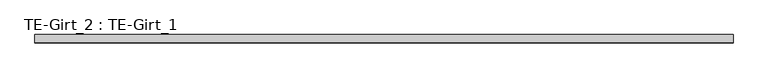
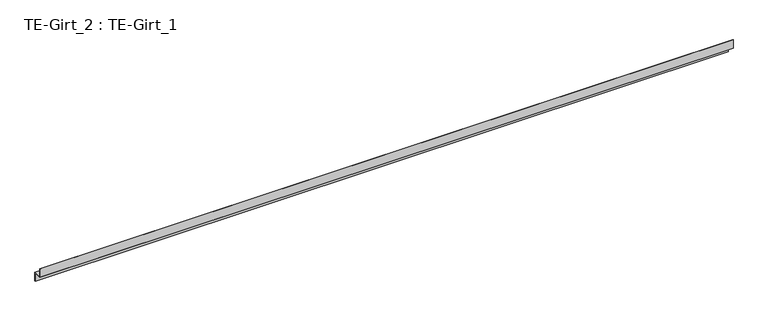
"""IFC4 building model written with IfcOpenShell, lengths in millimetres: proxy geometry, TE-Girt_2 : TE-Girt_1."""

from ifc_helpers import new_model, si_unit, frame, origin, place, context, project, spatial, polyline, outline, extrude, source, transform, mapped, element, save


def te_girt_2_te_girt_1_d8d35839(model_context):
    return source(origin(), model_context, "Body", "SweptSolid", [
        extrude(outline(polyline([(-531639.2163841, 1657.35), (-531639.2163841, 1619.25), (-531640.1093528, 1619.25), (-531640.1093528, 1656.4570312), (-531674.1249348, 1656.4570312), (-531674.1249348, 1694.5570312), (-531673.231966, 1694.5570312), (-531673.231966, 1657.35), (-531639.2163841, 1657.35)])), frame((587397.6434739, 0.0, 0.0), z_axis=(1.0, 0.0, 0.0), x_axis=(0.0, 1.0, 0.0)), (0.0, 0.0, 1.0), 2921.0),
    ])


if __name__ == "__main__":
    model = new_model("IFC4")
    model_context = context("Model", 3, world=origin())
    ifc_project = project(units=[si_unit("LENGTHUNIT", "METRE", prefix="MILLI")], contexts=[model_context])
    site = spatial("IfcSite", under=ifc_project)
    building = spatial("IfcBuilding", under=site)
    placement = place(None, origin())
    te_girt_2_te_girt_1_shape = te_girt_2_te_girt_1_d8d35839(model_context)
    element("IfcBuildingElementProxy", 1, Name="TE-Girt_2 : TE-Girt_1", ObjectType="TE-Girt_2 : TE-Girt_1", at=placement, inside=building, context=model_context, shape_type="MappedRepresentation", body=[
        mapped(te_girt_2_te_girt_1_shape, transform((0.0, 0.0, 0.0), x_axis=(1.0, 0.0, 0.0), y_axis=(0.0, 1.0, 0.0), z_axis=(0.0, 0.0, 1.0))),
    ])
    save(model, "model.ifc")

# Revit data of these elements
# Element 1 (IfcBuildingElementProxy, "TE-Girt_2 : TE-Girt_1")
#   Materials on its faces: "Z-FURRING, COLD-FORMED GALV."
# Materials
#   "Z-FURRING, COLD-FORMED GALV.": class "Generic", colour RGB 143 142 141, transparency 0, Cost = 0
